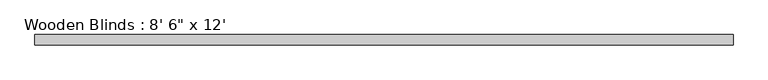
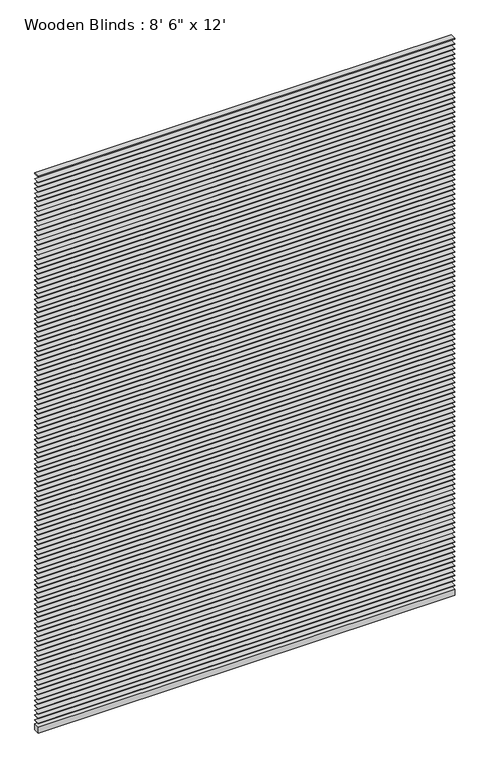
"""IFC4 building model written with IfcOpenShell, lengths in millimetres: furniture geometry."""

from ifc_helpers import new_model, si_unit, frame, origin, origin_with_axes, place, context, project, spatial, polyline, outline, extrude, source, transform, mapped, element, save


def furniture_73d83834(model_context):
    return source(origin(), model_context, "Body", "SweptSolid", [
        extrude(outline(polyline([(2590.8, 38.1), (2590.8, 0.0), (0.0, 0.0), (0.0, 38.1), (2590.8, 38.1)])), frame((0.0, 0.0, 3617.8790576), z_axis=(0.0, 0.0, 1.0), x_axis=(1.0, 0.0, 0.0)), (0.0, 0.0, 1.0), 3.175),
        extrude(outline(polyline([(2590.8, 38.1), (2590.8, 0.0), (0.0, 0.0), (0.0, 38.1), (2590.8, 38.1)])), frame((0.0, 0.0, 3586.1290576), z_axis=(0.0, 0.0, 1.0), x_axis=(1.0, 0.0, 0.0)), (0.0, 0.0, 1.0), 3.175),
        extrude(outline(polyline([(2590.8, 38.1), (2590.8, 0.0), (0.0, 0.0), (0.0, 38.1), (2590.8, 38.1)])), frame((0.0, 0.0, 3554.3790576), z_axis=(0.0, 0.0, 1.0), x_axis=(1.0, 0.0, 0.0)), (0.0, 0.0, 1.0), 3.175),
        extrude(outline(polyline([(2590.8, 38.1), (2590.8, 0.0), (0.0, 0.0), (0.0, 38.1), (2590.8, 38.1)])), frame((0.0, 0.0, 3522.6290576), z_axis=(0.0, 0.0, 1.0), x_axis=(1.0, 0.0, 0.0)), (0.0, 0.0, 1.0), 3.175),
        extrude(outline(polyline([(2590.8, 38.1), (2590.8, 0.0), (0.0, 0.0), (0.0, 38.1), (2590.8, 38.1)])), frame((0.0, 0.0, 3490.8790576), z_axis=(0.0, 0.0, 1.0), x_axis=(1.0, 0.0, 0.0)), (0.0, 0.0, 1.0), 3.175),
        extrude(outline(polyline([(2590.8, 38.1), (2590.8, 0.0), (0.0, 0.0), (0.0, 38.1), (2590.8, 38.1)])), frame((0.0, 0.0, 3459.1290576), z_axis=(0.0, 0.0, 1.0), x_axis=(1.0, 0.0, 0.0)), (0.0, 0.0, 1.0), 3.175),
        extrude(outline(polyline([(2590.8, 38.1), (2590.8, 0.0), (0.0, 0.0), (0.0, 38.1), (2590.8, 38.1)])), frame((0.0, 0.0, 3427.3790576), z_axis=(0.0, 0.0, 1.0), x_axis=(1.0, 0.0, 0.0)), (0.0, 0.0, 1.0), 3.175),
        extrude(outline(polyline([(2590.8, 38.1), (2590.8, 0.0), (0.0, 0.0), (0.0, 38.1), (2590.8, 38.1)])), frame((0.0, 0.0, 3395.6290576), z_axis=(0.0, 0.0, 1.0), x_axis=(1.0, 0.0, 0.0)), (0.0, 0.0, 1.0), 3.175),
        extrude(outline(polyline([(2590.8, 38.1), (2590.8, 0.0), (0.0, 0.0), (0.0, 38.1), (2590.8, 38.1)])), frame((0.0, 0.0, 3363.8790576), z_axis=(0.0, 0.0, 1.0), x_axis=(1.0, 0.0, 0.0)), (0.0, 0.0, 1.0), 3.175),
        extrude(outline(polyline([(2590.8, 38.1), (2590.8, 0.0), (0.0, 0.0), (0.0, 38.1), (2590.8, 38.1)])), frame((0.0, 0.0, 3332.1290576), z_axis=(0.0, 0.0, 1.0), x_axis=(1.0, 0.0, 0.0)), (0.0, 0.0, 1.0), 3.175),
        extrude(outline(polyline([(2590.8, 38.1), (2590.8, 0.0), (0.0, 0.0), (0.0, 38.1), (2590.8, 38.1)])), frame((0.0, 0.0, 3300.3790576), z_axis=(0.0, 0.0, 1.0), x_axis=(1.0, 0.0, 0.0)), (0.0, 0.0, 1.0), 3.175),
        extrude(outline(polyline([(2590.8, 38.1), (2590.8, 0.0), (0.0, 0.0), (0.0, 38.1), (2590.8, 38.1)])), frame((0.0, 0.0, 3268.6290576), z_axis=(0.0, 0.0, 1.0), x_axis=(1.0, 0.0, 0.0)), (0.0, 0.0, 1.0), 3.175),
        extrude(outline(polyline([(2590.8, 38.1), (2590.8, 0.0), (0.0, 0.0), (0.0, 38.1), (2590.8, 38.1)])), frame((0.0, 0.0, 3236.8790576), z_axis=(0.0, 0.0, 1.0), x_axis=(1.0, 0.0, 0.0)), (0.0, 0.0, 1.0), 3.175),
        extrude(outline(polyline([(2590.8, 38.1), (2590.8, 0.0), (0.0, 0.0), (0.0, 38.1), (2590.8, 38.1)])), frame((0.0, 0.0, 3205.1290576), z_axis=(0.0, 0.0, 1.0), x_axis=(1.0, 0.0, 0.0)), (0.0, 0.0, 1.0), 3.175),
        extrude(outline(polyline([(2590.8, 38.1), (2590.8, 0.0), (0.0, 0.0), (0.0, 38.1), (2590.8, 38.1)])), frame((0.0, 0.0, 3173.3790576), z_axis=(0.0, 0.0, 1.0), x_axis=(1.0, 0.0, 0.0)), (0.0, 0.0, 1.0), 3.175),
        extrude(outline(polyline([(2590.8, 38.1), (2590.8, 0.0), (0.0, 0.0), (0.0, 38.1), (2590.8, 38.1)])), frame((0.0, 0.0, 3141.6290576), z_axis=(0.0, 0.0, 1.0), x_axis=(1.0, 0.0, 0.0)), (0.0, 0.0, 1.0), 3.175),
        extrude(outline(polyline([(2590.8, 38.1), (2590.8, 0.0), (0.0, 0.0), (0.0, 38.1), (2590.8, 38.1)])), frame((0.0, 0.0, 3109.8790576), z_axis=(0.0, 0.0, 1.0), x_axis=(1.0, 0.0, 0.0)), (0.0, 0.0, 1.0), 3.175),
        extrude(outline(polyline([(2590.8, 38.1), (2590.8, 0.0), (0.0, 0.0), (0.0, 38.1), (2590.8, 38.1)])), frame((0.0, 0.0, 3078.1290576), z_axis=(0.0, 0.0, 1.0), x_axis=(1.0, 0.0, 0.0)), (0.0, 0.0, 1.0), 3.175),
        extrude(outline(polyline([(2590.8, 38.1), (2590.8, 0.0), (0.0, 0.0), (0.0, 38.1), (2590.8, 38.1)])), frame((0.0, 0.0, 3046.3790576), z_axis=(0.0, 0.0, 1.0), x_axis=(1.0, 0.0, 0.0)), (0.0, 0.0, 1.0), 3.175),
        extrude(outline(polyline([(2590.8, 38.1), (2590.8, 0.0), (0.0, 0.0), (0.0, 38.1), (2590.8, 38.1)])), frame((0.0, 0.0, 3014.6290576), z_axis=(0.0, 0.0, 1.0), x_axis=(1.0, 0.0, 0.0)), (0.0, 0.0, 1.0), 3.175),
        extrude(outline(polyline([(2590.8, 38.1), (2590.8, 0.0), (0.0, 0.0), (0.0, 38.1), (2590.8, 38.1)])), frame((0.0, 0.0, 2982.8790576), z_axis=(0.0, 0.0, 1.0), x_axis=(1.0, 0.0, 0.0)), (0.0, 0.0, 1.0), 3.175),
        extrude(outline(polyline([(2590.8, 38.1), (2590.8, 0.0), (0.0, 0.0), (0.0, 38.1), (2590.8, 38.1)])), frame((0.0, 0.0, 2951.1290576), z_axis=(0.0, 0.0, 1.0), x_axis=(1.0, 0.0, 0.0)), (0.0, 0.0, 1.0), 3.175),
        extrude(outline(polyline([(2590.8, 38.1), (2590.8, 0.0), (0.0, 0.0), (0.0, 38.1), (2590.8, 38.1)])), frame((0.0, 0.0, 2919.3790576), z_axis=(0.0, 0.0, 1.0), x_axis=(1.0, 0.0, 0.0)), (0.0, 0.0, 1.0), 3.175),
        extrude(outline(polyline([(2590.8, 38.1), (2590.8, 0.0), (0.0, 0.0), (0.0, 38.1), (2590.8, 38.1)])), frame((0.0, 0.0, 2887.6290576), z_axis=(0.0, 0.0, 1.0), x_axis=(1.0, 0.0, 0.0)), (0.0, 0.0, 1.0), 3.175),
        extrude(outline(polyline([(2590.8, 38.1), (2590.8, 0.0), (0.0, 0.0), (0.0, 38.1), (2590.8, 38.1)])), frame((0.0, 0.0, 2855.8790576), z_axis=(0.0, 0.0, 1.0), x_axis=(1.0, 0.0, 0.0)), (0.0, 0.0, 1.0), 3.175),
        extrude(outline(polyline([(2590.8, 38.1), (2590.8, 0.0), (0.0, 0.0), (0.0, 38.1), (2590.8, 38.1)])), frame((0.0, 0.0, 2824.1290576), z_axis=(0.0, 0.0, 1.0), x_axis=(1.0, 0.0, 0.0)), (0.0, 0.0, 1.0), 3.175),
        extrude(outline(polyline([(2590.8, 38.1), (2590.8, 0.0), (0.0, 0.0), (0.0, 38.1), (2590.8, 38.1)])), frame((0.0, 0.0, 2792.3790576), z_axis=(0.0, 0.0, 1.0), x_axis=(1.0, 0.0, 0.0)), (0.0, 0.0, 1.0), 3.175),
        extrude(outline(polyline([(2590.8, 38.1), (2590.8, 0.0), (0.0, 0.0), (0.0, 38.1), (2590.8, 38.1)])), frame((0.0, 0.0, 2760.6290576), z_axis=(0.0, 0.0, 1.0), x_axis=(1.0, 0.0, 0.0)), (0.0, 0.0, 1.0), 3.175),
        extrude(outline(polyline([(2590.8, 38.1), (2590.8, 0.0), (0.0, 0.0), (0.0, 38.1), (2590.8, 38.1)])), frame((0.0, 0.0, 2728.8790576), z_axis=(0.0, 0.0, 1.0), x_axis=(1.0, 0.0, 0.0)), (0.0, 0.0, 1.0), 3.175),
        extrude(outline(polyline([(2590.8, 38.1), (2590.8, 0.0), (0.0, 0.0), (0.0, 38.1), (2590.8, 38.1)])), frame((0.0, 0.0, 2697.1290576), z_axis=(0.0, 0.0, 1.0), x_axis=(1.0, 0.0, 0.0)), (0.0, 0.0, 1.0), 3.175),
        extrude(outline(polyline([(2590.8, 38.1), (2590.8, 0.0), (0.0, 0.0), (0.0, 38.1), (2590.8, 38.1)])), frame((0.0, 0.0, 2665.3790576), z_axis=(0.0, 0.0, 1.0), x_axis=(1.0, 0.0, 0.0)), (0.0, 0.0, 1.0), 3.175),
        extrude(outline(polyline([(2590.8, 38.1), (2590.8, 0.0), (0.0, 0.0), (0.0, 38.1), (2590.8, 38.1)])), frame((0.0, 0.0, 2633.6290576), z_axis=(0.0, 0.0, 1.0), x_axis=(1.0, 0.0, 0.0)), (0.0, 0.0, 1.0), 3.175),
        extrude(outline(polyline([(2590.8, 38.1), (2590.8, 0.0), (0.0, 0.0), (0.0, 38.1), (2590.8, 38.1)])), frame((0.0, 0.0, 2601.8790576), z_axis=(0.0, 0.0, 1.0), x_axis=(1.0, 0.0, 0.0)), (0.0, 0.0, 1.0), 3.175),
        extrude(outline(polyline([(2590.8, 38.1), (2590.8, 0.0), (0.0, 0.0), (0.0, 38.1), (2590.8, 38.1)])), frame((0.0, 0.0, 2570.1290576), z_axis=(0.0, 0.0, 1.0), x_axis=(1.0, 0.0, 0.0)), (0.0, 0.0, 1.0), 3.175),
        extrude(outline(polyline([(2590.8, 38.1), (2590.8, 0.0), (0.0, 0.0), (0.0, 38.1), (2590.8, 38.1)])), frame((0.0, 0.0, 2538.3790576), z_axis=(0.0, 0.0, 1.0), x_axis=(1.0, 0.0, 0.0)), (0.0, 0.0, 1.0), 3.175),
        extrude(outline(polyline([(2590.8, 38.1), (2590.8, 0.0), (0.0, 0.0), (0.0, 38.1), (2590.8, 38.1)])), frame((0.0, 0.0, 2506.6290576), z_axis=(0.0, 0.0, 1.0), x_axis=(1.0, 0.0, 0.0)), (0.0, 0.0, 1.0), 3.175),
        extrude(outline(polyline([(2590.8, 38.1), (2590.8, 0.0), (0.0, 0.0), (0.0, 38.1), (2590.8, 38.1)])), frame((0.0, 0.0, 2474.8790576), z_axis=(0.0, 0.0, 1.0), x_axis=(1.0, 0.0, 0.0)), (0.0, 0.0, 1.0), 3.175),
        extrude(outline(polyline([(2590.8, 38.1), (2590.8, 0.0), (0.0, 0.0), (0.0, 38.1), (2590.8, 38.1)])), frame((0.0, 0.0, 2443.1290576), z_axis=(0.0, 0.0, 1.0), x_axis=(1.0, 0.0, 0.0)), (0.0, 0.0, 1.0), 3.175),
        extrude(outline(polyline([(2590.8, 38.1), (2590.8, 0.0), (0.0, 0.0), (0.0, 38.1), (2590.8, 38.1)])), frame((0.0, 0.0, 2411.3790576), z_axis=(0.0, 0.0, 1.0), x_axis=(1.0, 0.0, 0.0)), (0.0, 0.0, 1.0), 3.175),
        extrude(outline(polyline([(2590.8, 38.1), (2590.8, 0.0), (0.0, 0.0), (0.0, 38.1), (2590.8, 38.1)])), frame((0.0, 0.0, 2379.6290576), z_axis=(0.0, 0.0, 1.0), x_axis=(1.0, 0.0, 0.0)), (0.0, 0.0, 1.0), 3.175),
        extrude(outline(polyline([(2590.8, 38.1), (2590.8, 0.0), (0.0, 0.0), (0.0, 38.1), (2590.8, 38.1)])), frame((0.0, 0.0, 2347.8790576), z_axis=(0.0, 0.0, 1.0), x_axis=(1.0, 0.0, 0.0)), (0.0, 0.0, 1.0), 3.175),
        extrude(outline(polyline([(2590.8, 38.1), (2590.8, 0.0), (0.0, 0.0), (0.0, 38.1), (2590.8, 38.1)])), frame((0.0, 0.0, 2316.1290576), z_axis=(0.0, 0.0, 1.0), x_axis=(1.0, 0.0, 0.0)), (0.0, 0.0, 1.0), 3.175),
        extrude(outline(polyline([(2590.8, 38.1), (2590.8, 0.0), (0.0, 0.0), (0.0, 38.1), (2590.8, 38.1)])), frame((0.0, 0.0, 2284.3790576), z_axis=(0.0, 0.0, 1.0), x_axis=(1.0, 0.0, 0.0)), (0.0, 0.0, 1.0), 3.175),
        extrude(outline(polyline([(2590.8, 38.1), (2590.8, 0.0), (0.0, 0.0), (0.0, 38.1), (2590.8, 38.1)])), frame((0.0, 0.0, 2252.6290576), z_axis=(0.0, 0.0, 1.0), x_axis=(1.0, 0.0, 0.0)), (0.0, 0.0, 1.0), 3.175),
        extrude(outline(polyline([(2590.8, 38.1), (2590.8, 0.0), (0.0, 0.0), (0.0, 38.1), (2590.8, 38.1)])), frame((0.0, 0.0, 2220.8790576), z_axis=(0.0, 0.0, 1.0), x_axis=(1.0, 0.0, 0.0)), (0.0, 0.0, 1.0), 3.175),
        extrude(outline(polyline([(2590.8, 38.1), (2590.8, 0.0), (0.0, 0.0), (0.0, 38.1), (2590.8, 38.1)])), frame((0.0, 0.0, 2189.1290576), z_axis=(0.0, 0.0, 1.0), x_axis=(1.0, 0.0, 0.0)), (0.0, 0.0, 1.0), 3.175),
        extrude(outline(polyline([(2590.8, 38.1), (2590.8, 0.0), (0.0, 0.0), (0.0, 38.1), (2590.8, 38.1)])), frame((0.0, 0.0, 2157.3790576), z_axis=(0.0, 0.0, 1.0), x_axis=(1.0, 0.0, 0.0)), (0.0, 0.0, 1.0), 3.175),
        extrude(outline(polyline([(2590.8, 38.1), (2590.8, 0.0), (0.0, 0.0), (0.0, 38.1), (2590.8, 38.1)])), frame((0.0, 0.0, 2125.6290576), z_axis=(0.0, 0.0, 1.0), x_axis=(1.0, 0.0, 0.0)), (0.0, 0.0, 1.0), 3.175),
        extrude(outline(polyline([(2590.8, 38.1), (2590.8, 0.0), (0.0, 0.0), (0.0, 38.1), (2590.8, 38.1)])), frame((0.0, 0.0, 2093.8790576), z_axis=(0.0, 0.0, 1.0), x_axis=(1.0, 0.0, 0.0)), (0.0, 0.0, 1.0), 3.175),
        extrude(outline(polyline([(2590.8, 38.1), (2590.8, 0.0), (0.0, 0.0), (0.0, 38.1), (2590.8, 38.1)])), frame((0.0, 0.0, 2062.1290576), z_axis=(0.0, 0.0, 1.0), x_axis=(1.0, 0.0, 0.0)), (0.0, 0.0, 1.0), 3.175),
        extrude(outline(polyline([(2590.8, 38.1), (2590.8, 0.0), (0.0, 0.0), (0.0, 38.1), (2590.8, 38.1)])), frame((0.0, 0.0, 2030.3790576), z_axis=(0.0, 0.0, 1.0), x_axis=(1.0, 0.0, 0.0)), (0.0, 0.0, 1.0), 3.175),
        extrude(outline(polyline([(2590.8, 38.1), (2590.8, 0.0), (0.0, 0.0), (0.0, 38.1), (2590.8, 38.1)])), frame((0.0, 0.0, 1998.6290576), z_axis=(0.0, 0.0, 1.0), x_axis=(1.0, 0.0, 0.0)), (0.0, 0.0, 1.0), 3.175),
        extrude(outline(polyline([(2590.8, 38.1), (2590.8, 0.0), (0.0, 0.0), (0.0, 38.1), (2590.8, 38.1)])), frame((0.0, 0.0, 1966.8790576), z_axis=(0.0, 0.0, 1.0), x_axis=(1.0, 0.0, 0.0)), (0.0, 0.0, 1.0), 3.175),
        extrude(outline(polyline([(2590.8, 38.1), (2590.8, 0.0), (0.0, 0.0), (0.0, 38.1), (2590.8, 38.1)])), frame((0.0, 0.0, 1935.1290576), z_axis=(0.0, 0.0, 1.0), x_axis=(1.0, 0.0, 0.0)), (0.0, 0.0, 1.0), 3.175),
        extrude(outline(polyline([(2590.8, 38.1), (2590.8, 0.0), (0.0, 0.0), (0.0, 38.1), (2590.8, 38.1)])), frame((0.0, 0.0, 1903.3790576), z_axis=(0.0, 0.0, 1.0), x_axis=(1.0, 0.0, 0.0)), (0.0, 0.0, 1.0), 3.175),
        extrude(outline(polyline([(2590.8, 38.1), (2590.8, 0.0), (0.0, 0.0), (0.0, 38.1), (2590.8, 38.1)])), frame((0.0, 0.0, 1871.6290576), z_axis=(0.0, 0.0, 1.0), x_axis=(1.0, 0.0, 0.0)), (0.0, 0.0, 1.0), 3.175),
        extrude(outline(polyline([(2590.8, 38.1), (2590.8, 0.0), (0.0, 0.0), (0.0, 38.1), (2590.8, 38.1)])), frame((0.0, 0.0, 1839.8790576), z_axis=(0.0, 0.0, 1.0), x_axis=(1.0, 0.0, 0.0)), (0.0, 0.0, 1.0), 3.175),
        extrude(outline(polyline([(2590.8, 38.1), (2590.8, 0.0), (0.0, 0.0), (0.0, 38.1), (2590.8, 38.1)])), frame((0.0, 0.0, 1808.1290576), z_axis=(0.0, 0.0, 1.0), x_axis=(1.0, 0.0, 0.0)), (0.0, 0.0, 1.0), 3.175),
        extrude(outline(polyline([(2590.8, 38.1), (2590.8, 0.0), (0.0, 0.0), (0.0, 38.1), (2590.8, 38.1)])), frame((0.0, 0.0, 1776.3790576), z_axis=(0.0, 0.0, 1.0), x_axis=(1.0, 0.0, 0.0)), (0.0, 0.0, 1.0), 3.175),
        extrude(outline(polyline([(2590.8, 38.1), (2590.8, 0.0), (0.0, 0.0), (0.0, 38.1), (2590.8, 38.1)])), frame((0.0, 0.0, 1744.6290576), z_axis=(0.0, 0.0, 1.0), x_axis=(1.0, 0.0, 0.0)), (0.0, 0.0, 1.0), 3.175),
        extrude(outline(polyline([(2590.8, 38.1), (2590.8, 0.0), (0.0, 0.0), (0.0, 38.1), (2590.8, 38.1)])), frame((0.0, 0.0, 1712.8790576), z_axis=(0.0, 0.0, 1.0), x_axis=(1.0, 0.0, 0.0)), (0.0, 0.0, 1.0), 3.175),
        extrude(outline(polyline([(2590.8, 38.1), (2590.8, 0.0), (0.0, 0.0), (0.0, 38.1), (2590.8, 38.1)])), frame((0.0, 0.0, 1681.1290576), z_axis=(0.0, 0.0, 1.0), x_axis=(1.0, 0.0, 0.0)), (0.0, 0.0, 1.0), 3.175),
        extrude(outline(polyline([(2590.8, 38.1), (2590.8, 0.0), (0.0, 0.0), (0.0, 38.1), (2590.8, 38.1)])), frame((0.0, 0.0, 1649.3790576), z_axis=(0.0, 0.0, 1.0), x_axis=(1.0, 0.0, 0.0)), (0.0, 0.0, 1.0), 3.175),
        extrude(outline(polyline([(2590.8, 38.1), (2590.8, 0.0), (0.0, 0.0), (0.0, 38.1), (2590.8, 38.1)])), frame((0.0, 0.0, 1617.6290576), z_axis=(0.0, 0.0, 1.0), x_axis=(1.0, 0.0, 0.0)), (0.0, 0.0, 1.0), 3.175),
        extrude(outline(polyline([(2590.8, 38.1), (2590.8, 0.0), (0.0, 0.0), (0.0, 38.1), (2590.8, 38.1)])), frame((0.0, 0.0, 1585.8790576), z_axis=(0.0, 0.0, 1.0), x_axis=(1.0, 0.0, 0.0)), (0.0, 0.0, 1.0), 3.175),
        extrude(outline(polyline([(2590.8, 38.1), (2590.8, 0.0), (0.0, 0.0), (0.0, 38.1), (2590.8, 38.1)])), frame((0.0, 0.0, 1554.1290576), z_axis=(0.0, 0.0, 1.0), x_axis=(1.0, 0.0, 0.0)), (0.0, 0.0, 1.0), 3.175),
        extrude(outline(polyline([(2590.8, 38.1), (2590.8, 0.0), (0.0, 0.0), (0.0, 38.1), (2590.8, 38.1)])), frame((0.0, 0.0, 1522.3790576), z_axis=(0.0, 0.0, 1.0), x_axis=(1.0, 0.0, 0.0)), (0.0, 0.0, 1.0), 3.175),
        extrude(outline(polyline([(2590.8, 38.1), (2590.8, 0.0), (0.0, 0.0), (0.0, 38.1), (2590.8, 38.1)])), frame((0.0, 0.0, 1490.6290576), z_axis=(0.0, 0.0, 1.0), x_axis=(1.0, 0.0, 0.0)), (0.0, 0.0, 1.0), 3.175),
        extrude(outline(polyline([(2590.8, 38.1), (2590.8, 0.0), (0.0, 0.0), (0.0, 38.1), (2590.8, 38.1)])), frame((0.0, 0.0, 1458.8790576), z_axis=(0.0, 0.0, 1.0), x_axis=(1.0, 0.0, 0.0)), (0.0, 0.0, 1.0), 3.175),
        extrude(outline(polyline([(2590.8, 38.1), (2590.8, 0.0), (0.0, 0.0), (0.0, 38.1), (2590.8, 38.1)])), frame((0.0, 0.0, 1427.1290576), z_axis=(0.0, 0.0, 1.0), x_axis=(1.0, 0.0, 0.0)), (0.0, 0.0, 1.0), 3.175),
        extrude(outline(polyline([(2590.8, 38.1), (2590.8, 0.0), (0.0, 0.0), (0.0, 38.1), (2590.8, 38.1)])), frame((0.0, 0.0, 1395.3790576), z_axis=(0.0, 0.0, 1.0), x_axis=(1.0, 0.0, 0.0)), (0.0, 0.0, 1.0), 3.175),
        extrude(outline(polyline([(2590.8, 38.1), (2590.8, 0.0), (0.0, 0.0), (0.0, 38.1), (2590.8, 38.1)])), frame((0.0, 0.0, 1363.6290576), z_axis=(0.0, 0.0, 1.0), x_axis=(1.0, 0.0, 0.0)), (0.0, 0.0, 1.0), 3.175),
        extrude(outline(polyline([(2590.8, 38.1), (2590.8, 0.0), (0.0, 0.0), (0.0, 38.1), (2590.8, 38.1)])), frame((0.0, 0.0, 1331.8790576), z_axis=(0.0, 0.0, 1.0), x_axis=(1.0, 0.0, 0.0)), (0.0, 0.0, 1.0), 3.175),
        extrude(outline(polyline([(2590.8, 38.1), (2590.8, 0.0), (0.0, 0.0), (0.0, 38.1), (2590.8, 38.1)])), frame((0.0, 0.0, 1300.1290576), z_axis=(0.0, 0.0, 1.0), x_axis=(1.0, 0.0, 0.0)), (0.0, 0.0, 1.0), 3.175),
        extrude(outline(polyline([(2590.8, 38.1), (2590.8, 0.0), (0.0, 0.0), (0.0, 38.1), (2590.8, 38.1)])), frame((0.0, 0.0, 1268.3790576), z_axis=(0.0, 0.0, 1.0), x_axis=(1.0, 0.0, 0.0)), (0.0, 0.0, 1.0), 3.175),
        extrude(outline(polyline([(2590.8, 38.1), (2590.8, 0.0), (0.0, 0.0), (0.0, 38.1), (2590.8, 38.1)])), frame((0.0, 0.0, 1236.6290576), z_axis=(0.0, 0.0, 1.0), x_axis=(1.0, 0.0, 0.0)), (0.0, 0.0, 1.0), 3.175),
        extrude(outline(polyline([(2590.8, 38.1), (2590.8, 0.0), (0.0, 0.0), (0.0, 38.1), (2590.8, 38.1)])), frame((0.0, 0.0, 1204.8790576), z_axis=(0.0, 0.0, 1.0), x_axis=(1.0, 0.0, 0.0)), (0.0, 0.0, 1.0), 3.175),
        extrude(outline(polyline([(2590.8, 38.1), (2590.8, 0.0), (0.0, 0.0), (0.0, 38.1), (2590.8, 38.1)])), frame((0.0, 0.0, 1173.1290576), z_axis=(0.0, 0.0, 1.0), x_axis=(1.0, 0.0, 0.0)), (0.0, 0.0, 1.0), 3.175),
        extrude(outline(polyline([(2590.8, 38.1), (2590.8, 0.0), (0.0, 0.0), (0.0, 38.1), (2590.8, 38.1)])), frame((0.0, 0.0, 1141.3790576), z_axis=(0.0, 0.0, 1.0), x_axis=(1.0, 0.0, 0.0)), (0.0, 0.0, 1.0), 3.175),
        extrude(outline(polyline([(2590.8, 38.1), (2590.8, 0.0), (0.0, 0.0), (0.0, 38.1), (2590.8, 38.1)])), frame((0.0, 0.0, 1109.6290576), z_axis=(0.0, 0.0, 1.0), x_axis=(1.0, 0.0, 0.0)), (0.0, 0.0, 1.0), 3.175),
        extrude(outline(polyline([(2590.8, 38.1), (2590.8, 0.0), (0.0, 0.0), (0.0, 38.1), (2590.8, 38.1)])), frame((0.0, 0.0, 1077.8790576), z_axis=(0.0, 0.0, 1.0), x_axis=(1.0, 0.0, 0.0)), (0.0, 0.0, 1.0), 3.175),
        extrude(outline(polyline([(2590.8, 38.1), (2590.8, 0.0), (0.0, 0.0), (0.0, 38.1), (2590.8, 38.1)])), frame((0.0, 0.0, 1046.1290576), z_axis=(0.0, 0.0, 1.0), x_axis=(1.0, 0.0, 0.0)), (0.0, 0.0, 1.0), 3.175),
        extrude(outline(polyline([(2590.8, 38.1), (2590.8, 0.0), (0.0, 0.0), (0.0, 38.1), (2590.8, 38.1)])), frame((0.0, 0.0, 1014.3790576), z_axis=(0.0, 0.0, 1.0), x_axis=(1.0, 0.0, 0.0)), (0.0, 0.0, 1.0), 3.175),
        extrude(outline(polyline([(2590.8, 38.1), (2590.8, 0.0), (0.0, 0.0), (0.0, 38.1), (2590.8, 38.1)])), frame((0.0, 0.0, 982.6290576), z_axis=(0.0, 0.0, 1.0), x_axis=(1.0, 0.0, 0.0)), (0.0, 0.0, 1.0), 3.175),
        extrude(outline(polyline([(2590.8, 38.1), (2590.8, 0.0), (0.0, 0.0), (0.0, 38.1), (2590.8, 38.1)])), frame((0.0, 0.0, 950.8790576), z_axis=(0.0, 0.0, 1.0), x_axis=(1.0, 0.0, 0.0)), (0.0, 0.0, 1.0), 3.175),
        extrude(outline(polyline([(2590.8, 38.1), (2590.8, 0.0), (0.0, 0.0), (0.0, 38.1), (2590.8, 38.1)])), frame((0.0, 0.0, 919.1290576), z_axis=(0.0, 0.0, 1.0), x_axis=(1.0, 0.0, 0.0)), (0.0, 0.0, 1.0), 3.175),
        extrude(outline(polyline([(2590.8, 38.1), (2590.8, 0.0), (0.0, 0.0), (0.0, 38.1), (2590.8, 38.1)])), frame((0.0, 0.0, 887.3790576), z_axis=(0.0, 0.0, 1.0), x_axis=(1.0, 0.0, 0.0)), (0.0, 0.0, 1.0), 3.175),
        extrude(outline(polyline([(2590.8, 38.1), (2590.8, 0.0), (0.0, 0.0), (0.0, 38.1), (2590.8, 38.1)])), frame((0.0, 0.0, 855.6290576), z_axis=(0.0, 0.0, 1.0), x_axis=(1.0, 0.0, 0.0)), (0.0, 0.0, 1.0), 3.175),
        extrude(outline(polyline([(2590.8, 38.1), (2590.8, 0.0), (0.0, 0.0), (0.0, 38.1), (2590.8, 38.1)])), frame((0.0, 0.0, 823.8790576), z_axis=(0.0, 0.0, 1.0), x_axis=(1.0, 0.0, 0.0)), (0.0, 0.0, 1.0), 3.175),
        extrude(outline(polyline([(2590.8, 38.1), (2590.8, 0.0), (0.0, 0.0), (0.0, 38.1), (2590.8, 38.1)])), frame((0.0, 0.0, 792.1290576), z_axis=(0.0, 0.0, 1.0), x_axis=(1.0, 0.0, 0.0)), (0.0, 0.0, 1.0), 3.175),
        extrude(outline(polyline([(2590.8, 38.1), (2590.8, 0.0), (0.0, 0.0), (0.0, 38.1), (2590.8, 38.1)])), frame((0.0, 0.0, 760.3790576), z_axis=(0.0, 0.0, 1.0), x_axis=(1.0, 0.0, 0.0)), (0.0, 0.0, 1.0), 3.175),
        extrude(outline(polyline([(2590.8, 38.1), (2590.8, 0.0), (0.0, 0.0), (0.0, 38.1), (2590.8, 38.1)])), frame((0.0, 0.0, 728.6290576), z_axis=(0.0, 0.0, 1.0), x_axis=(1.0, 0.0, 0.0)), (0.0, 0.0, 1.0), 3.175),
        extrude(outline(polyline([(2590.8, 38.1), (2590.8, 0.0), (0.0, 0.0), (0.0, 38.1), (2590.8, 38.1)])), frame((0.0, 0.0, 696.8790576), z_axis=(0.0, 0.0, 1.0), x_axis=(1.0, 0.0, 0.0)), (0.0, 0.0, 1.0), 3.175),
        extrude(outline(polyline([(2590.8, 38.1), (2590.8, 0.0), (0.0, 0.0), (0.0, 38.1), (2590.8, 38.1)])), frame((0.0, 0.0, 665.1290576), z_axis=(0.0, 0.0, 1.0), x_axis=(1.0, 0.0, 0.0)), (0.0, 0.0, 1.0), 3.175),
        extrude(outline(polyline([(2590.8, 38.1), (2590.8, 0.0), (0.0, 0.0), (0.0, 38.1), (2590.8, 38.1)])), frame((0.0, 0.0, 633.3790576), z_axis=(0.0, 0.0, 1.0), x_axis=(1.0, 0.0, 0.0)), (0.0, 0.0, 1.0), 3.175),
        extrude(outline(polyline([(2590.8, 38.1), (2590.8, 0.0), (0.0, 0.0), (0.0, 38.1), (2590.8, 38.1)])), frame((0.0, 0.0, 601.6290576), z_axis=(0.0, 0.0, 1.0), x_axis=(1.0, 0.0, 0.0)), (0.0, 0.0, 1.0), 3.175),
        extrude(outline(polyline([(2590.8, 38.1), (2590.8, 0.0), (0.0, 0.0), (0.0, 38.1), (2590.8, 38.1)])), frame((0.0, 0.0, 569.8790576), z_axis=(0.0, 0.0, 1.0), x_axis=(1.0, 0.0, 0.0)), (0.0, 0.0, 1.0), 3.175),
        extrude(outline(polyline([(2590.8, 38.1), (2590.8, 0.0), (0.0, 0.0), (0.0, 38.1), (2590.8, 38.1)])), frame((0.0, 0.0, 538.1290576), z_axis=(0.0, 0.0, 1.0), x_axis=(1.0, 0.0, 0.0)), (0.0, 0.0, 1.0), 3.175),
        extrude(outline(polyline([(2590.8, 38.1), (2590.8, 0.0), (0.0, 0.0), (0.0, 38.1), (2590.8, 38.1)])), frame((0.0, 0.0, 506.3790576), z_axis=(0.0, 0.0, 1.0), x_axis=(1.0, 0.0, 0.0)), (0.0, 0.0, 1.0), 3.175),
        extrude(outline(polyline([(2590.8, 38.1), (2590.8, 0.0), (0.0, 0.0), (0.0, 38.1), (2590.8, 38.1)])), frame((0.0, 0.0, 474.6290576), z_axis=(0.0, 0.0, 1.0), x_axis=(1.0, 0.0, 0.0)), (0.0, 0.0, 1.0), 3.175),
        extrude(outline(polyline([(2590.8, 38.1), (2590.8, 0.0), (0.0, 0.0), (0.0, 38.1), (2590.8, 38.1)])), frame((0.0, 0.0, 442.8790576), z_axis=(0.0, 0.0, 1.0), x_axis=(1.0, 0.0, 0.0)), (0.0, 0.0, 1.0), 3.175),
        extrude(outline(polyline([(2590.8, 38.1), (2590.8, 0.0), (0.0, 0.0), (0.0, 38.1), (2590.8, 38.1)])), frame((0.0, 0.0, 411.1290576), z_axis=(0.0, 0.0, 1.0), x_axis=(1.0, 0.0, 0.0)), (0.0, 0.0, 1.0), 3.175),
        extrude(outline(polyline([(2590.8, 38.1), (2590.8, 0.0), (0.0, 0.0), (0.0, 38.1), (2590.8, 38.1)])), frame((0.0, 0.0, 379.3790576), z_axis=(0.0, 0.0, 1.0), x_axis=(1.0, 0.0, 0.0)), (0.0, 0.0, 1.0), 3.175),
        extrude(outline(polyline([(2590.8, 38.1), (2590.8, 0.0), (0.0, 0.0), (0.0, 38.1), (2590.8, 38.1)])), frame((0.0, 0.0, 347.6290576), z_axis=(0.0, 0.0, 1.0), x_axis=(1.0, 0.0, 0.0)), (0.0, 0.0, 1.0), 3.175),
        extrude(outline(polyline([(2590.8, 38.1), (2590.8, 0.0), (0.0, 0.0), (0.0, 38.1), (2590.8, 38.1)])), frame((0.0, 0.0, 315.8790576), z_axis=(0.0, 0.0, 1.0), x_axis=(1.0, 0.0, 0.0)), (0.0, 0.0, 1.0), 3.175),
        extrude(outline(polyline([(2590.8, 38.1), (2590.8, 0.0), (0.0, 0.0), (0.0, 38.1), (2590.8, 38.1)])), frame((0.0, 0.0, 284.1290576), z_axis=(0.0, 0.0, 1.0), x_axis=(1.0, 0.0, 0.0)), (0.0, 0.0, 1.0), 3.175),
        extrude(outline(polyline([(2590.8, 38.1), (2590.8, 0.0), (0.0, 0.0), (0.0, 38.1), (2590.8, 38.1)])), frame((0.0, 0.0, 252.3790576), z_axis=(0.0, 0.0, 1.0), x_axis=(1.0, 0.0, 0.0)), (0.0, 0.0, 1.0), 3.175),
        extrude(outline(polyline([(2590.8, 38.1), (2590.8, 0.0), (0.0, 0.0), (0.0, 38.1), (2590.8, 38.1)])), frame((0.0, 0.0, 220.6290576), z_axis=(0.0, 0.0, 1.0), x_axis=(1.0, 0.0, 0.0)), (0.0, 0.0, 1.0), 3.175),
        extrude(outline(polyline([(2590.8, 38.1), (2590.8, 0.0), (0.0, 0.0), (0.0, 38.1), (2590.8, 38.1)])), frame((0.0, 0.0, 188.8790576), z_axis=(0.0, 0.0, 1.0), x_axis=(1.0, 0.0, 0.0)), (0.0, 0.0, 1.0), 3.175),
        extrude(outline(polyline([(2590.8, 38.1), (2590.8, 0.0), (0.0, 0.0), (0.0, 38.1), (2590.8, 38.1)])), frame((0.0, 0.0, 157.1290576), z_axis=(0.0, 0.0, 1.0), x_axis=(1.0, 0.0, 0.0)), (0.0, 0.0, 1.0), 3.175),
        extrude(outline(polyline([(2590.8, 38.1), (2590.8, 0.0), (0.0, 0.0), (0.0, 38.1), (2590.8, 38.1)])), frame((0.0, 0.0, 125.3790576), z_axis=(0.0, 0.0, 1.0), x_axis=(1.0, 0.0, 0.0)), (0.0, 0.0, 1.0), 3.175),
        extrude(outline(polyline([(2590.8, 38.1), (2590.8, 0.0), (0.0, 0.0), (0.0, 38.1), (2590.8, 38.1)])), frame((0.0, 0.0, 93.6290576), z_axis=(0.0, 0.0, 1.0), x_axis=(1.0, 0.0, 0.0)), (0.0, 0.0, 1.0), 3.175),
        extrude(outline(polyline([(2590.8, 38.1), (2590.8, 0.0), (0.0, 0.0), (0.0, 38.1), (2590.8, 38.1)])), frame((0.0, 0.0, 61.8790576), z_axis=(0.0, 0.0, 1.0), x_axis=(1.0, 0.0, 0.0)), (0.0, 0.0, 1.0), 3.175),
        extrude(outline(polyline([(2590.8, 38.1), (2590.8, 0.0), (0.0, 0.0), (0.0, 38.1), (2590.8, 38.1)])), frame((0.0, 0.0, 3651.25), z_axis=(0.0, 0.0, 1.0), x_axis=(1.0, 0.0, 0.0)), (0.0, 0.0, 1.0), 6.35),
        extrude(outline(polyline([(2590.8, 38.1), (2590.8, 0.0), (0.0, 0.0), (0.0, 38.1), (2590.8, 38.1)])), origin_with_axes(), (0.0, 0.0, 1.0), 38.1),
    ])


if __name__ == "__main__":
    model = new_model("IFC4")
    model_context = context("Model", 3, world=origin())
    ifc_project = project(units=[si_unit("LENGTHUNIT", "METRE", prefix="MILLI")], contexts=[model_context])
    site = spatial("IfcSite", under=ifc_project)
    building = spatial("IfcBuilding", under=site)
    placement = place(None, origin())
    furniture_shape = furniture_73d83834(model_context)
    element("IfcFurniture", 1, ObjectType="Wooden Blinds : 8' 6\" x 12'", at=placement, inside=building, context=model_context, shape_type="MappedRepresentation", body=[
        mapped(furniture_shape, transform((0.0, 0.0, 0.0), x_axis=(1.0, 0.0, 0.0), y_axis=(0.0, 1.0, 0.0), z_axis=(0.0, 0.0, 1.0))),
    ])
    save(model, "model.ifc")

# Revit data of these elements
# Type "Wooden Blinds : 8' 6\" x 12'"
#   Width = 8' - 6"
#   Slat Thickness = 0' - 0 1/8"
#   Height = 12' - 0"
#   Depth = 0' - 1 1/2"
#   Default Elevation = 4' - 0"
#   Blind Rotation = 90.00°
#   Number of Slats = 113
#   Slat = Metal - Chrome
#   Frame = Metal - Chrome
#   Assembly Code = ""
# Element 1 (IfcFurniture, "Wooden Blinds : 8' 6\" x 12'")
#   Materials on its faces: "Metal - Chrome"
# Materials
#   "Metal - Chrome": class "Metal", colour RGB 244 244 244, transparency 0, Comments = "Rendering appearance not upgraded Rendering appearance not upgraded ", Description = "Chrome"
